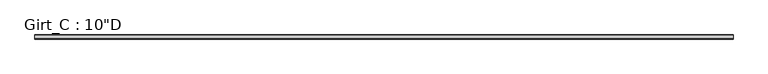
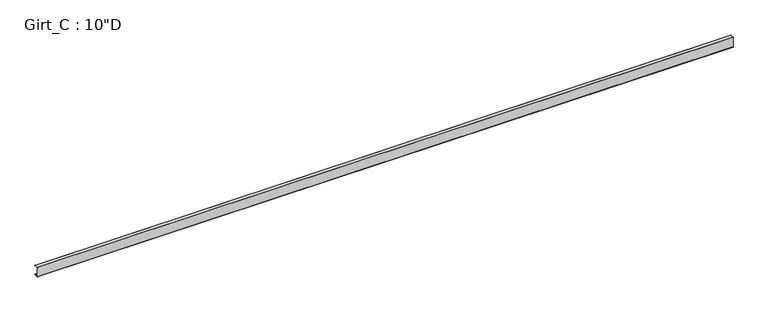
"""IFC4 building model written with IfcOpenShell, lengths in millimetres: beam geometry."""

import ifcopenshell
import ifcopenshell.guid

model = None  # the IFC model being written
_history = None  # IfcOwnerHistory: only IFC2X3 demands one
_inside = {}  # id of a spatial element -> (the spatial element, [elements in it])
_under = {}  # id of a project, library or spatial element -> (it, [spatial elements below it])
_declared = {}  # id of a project -> (the project, [libraries it declares])
_typed = {}  # id of a type object -> (the type object, [elements of that type])
_made_of = {}  # id of a material, layer set ... -> (it, [elements and type objects made of it])


def new_model(schema):
    """Start an empty IFC model of exactly this schema.

    Asked for "IFC4X3", IfcOpenShell would pick the latest addendum, in which some entities
    have other attributes; the version numbers below select the first issue.
    IFC2X3 requires an IfcOwnerHistory on every rooted entity: one is made here for all.
    """
    global model, _history
    if schema == "IFC4X3":
        model = ifcopenshell.file(schema_version=(4, 3, 0, 0))
    else:
        model = ifcopenshell.file(schema=schema)
    _inside.clear()
    _under.clear()
    _declared.clear()
    _typed.clear()
    _made_of.clear()
    _history = None
    if model.schema == "IFC2X3":
        org = make("IfcOrganization", Name="unknown")
        user = make(
            "IfcPersonAndOrganization",
            ThePerson=make("IfcPerson", FamilyName="unknown"),
            TheOrganization=org,
        )
        app = make(
            "IfcApplication",
            ApplicationDeveloper=org,
            Version="unknown",
            ApplicationFullName="unknown",
            ApplicationIdentifier="unknown",
        )
        _history = make(
            "IfcOwnerHistory",
            OwningUser=user,
            OwningApplication=app,
            ChangeAction="ADDED",
            CreationDate=0,
        )
    return model


def make(cls, **values):
    """One entity of the class cls with the attributes given. An attribute that is None is left unset."""
    return model.create_entity(
        cls, **{name: value for name, value in values.items() if value is not None}
    )


def rooted(cls, **values):
    """An entity with a GlobalId (a new one), such as an element, a storey or a relation."""
    return make(cls, GlobalId=ifcopenshell.guid.new(), OwnerHistory=_history, **values)


def si_unit(unit_type, name, prefix=None):
    """IfcSIUnit, for example si_unit("LENGTHUNIT", "METRE", prefix="MILLI")."""
    return make("IfcSIUnit", UnitType=unit_type, Prefix=prefix, Name=name)


def assignment(units):
    """IfcUnitAssignment: the units of a project."""
    return None if units is None else make("IfcUnitAssignment", Units=units)


def point(xyz):
    """IfcCartesianPoint."""
    return None if xyz is None else make("IfcCartesianPoint", Coordinates=xyz)


def direction(xyz):
    """IfcDirection."""
    return None if xyz is None else make("IfcDirection", DirectionRatios=xyz)


def frame(location, z_axis=None, x_axis=None):
    """IfcAxis2Placement3D, a coordinate frame: its origin and axes. An axis left out is left unset."""
    return make(
        "IfcAxis2Placement3D",
        Location=point(location),
        Axis=direction(z_axis),
        RefDirection=direction(x_axis),
    )


def frame_2d(location, x_axis=None):
    """IfcAxis2Placement2D, a coordinate frame in the plane: its origin and x axis."""
    return make(
        "IfcAxis2Placement2D", Location=point(location), RefDirection=direction(x_axis)
    )


def origin():
    """The frame at (0, 0, 0) with its axes left unset."""
    return frame((0.0, 0.0, 0.0))


def place(relative_to, where):
    """IfcLocalPlacement: puts the frame where relative to a parent placement (None: the world)."""
    return make(
        "IfcLocalPlacement", PlacementRelTo=relative_to, RelativePlacement=where
    )


def context(
    kind, dimensions, precision=None, world=None, true_north=None, identifier=None
):
    """IfcGeometricRepresentationContext, for example the 3D "Model" context."""
    return make(
        "IfcGeometricRepresentationContext",
        ContextIdentifier=identifier,
        ContextType=kind,
        CoordinateSpaceDimension=dimensions,
        Precision=precision,
        WorldCoordinateSystem=world,
        TrueNorth=true_north,
    )


def project(units=None, contexts=None):
    """IfcProject with its units and contexts."""
    return rooted(
        "IfcProject",
        Name="project",
        RepresentationContexts=contexts,
        UnitsInContext=assignment(units),
    )


def spatial(cls, under=None, at=None, **own):
    """A site, building, storey or space (cls), placed at a placement, below another one or the project."""
    s = rooted(cls, ObjectPlacement=at, **own)
    if under is not None:
        _under.setdefault(under.id(), (under, []))[1].append(s)
    return s


def polyline(points):
    """IfcPolyline through the points."""
    return make("IfcPolyline", Points=[point(p) for p in points])


def circle_curve(where, radius):
    """IfcCircle in the frame where."""
    return make("IfcCircle", Position=where, Radius=radius)


def trimmed(basis, trim1, trim2, sense, master):
    """IfcTrimmedCurve: the piece of a basis curve between two trims."""
    return make(
        "IfcTrimmedCurve",
        BasisCurve=basis,
        Trim1=trim1,
        Trim2=trim2,
        SenseAgreement=sense,
        MasterRepresentation=master,
    )


def segment(curve, same_sense, transition):
    """IfcCompositeCurveSegment."""
    return make(
        "IfcCompositeCurveSegment",
        Transition=transition,
        SameSense=same_sense,
        ParentCurve=curve,
    )


def composite_curve(segments, self_intersect=None):
    """IfcCompositeCurve: segments joined end to end."""
    return make("IfcCompositeCurve", Segments=segments, SelfIntersect=self_intersect)


def outline(outer, holes=None, kind="AREA"):
    """IfcArbitraryClosedProfileDef: a profile drawn as a closed curve; with holes, ...WithVoids."""
    if holes is None:
        return make("IfcArbitraryClosedProfileDef", ProfileType=kind, OuterCurve=outer)
    return make(
        "IfcArbitraryProfileDefWithVoids",
        ProfileType=kind,
        OuterCurve=outer,
        InnerCurves=holes,
    )


def extrude(swept, where, along, depth):
    """IfcExtrudedAreaSolid: the profile swept, set in the frame where, extruded along a direction by depth."""
    return make(
        "IfcExtrudedAreaSolid",
        SweptArea=swept,
        Position=where,
        ExtrudedDirection=direction(along),
        Depth=depth,
    )


def shape(context_of_items, identifier, shape_type, items):
    """IfcShapeRepresentation: the items that make up one representation, for example the "Body"."""
    return make(
        "IfcShapeRepresentation",
        ContextOfItems=context_of_items,
        RepresentationIdentifier=identifier,
        RepresentationType=shape_type,
        Items=items,
    )


def source(mapping_origin, context_of_items, identifier, shape_type, items):
    """IfcRepresentationMap: a shape defined once, which mapped items show again and again."""
    return make(
        "IfcRepresentationMap",
        MappingOrigin=mapping_origin,
        MappedRepresentation=shape(context_of_items, identifier, shape_type, items),
    )


def transform(
    local_origin,
    x_axis=None,
    y_axis=None,
    z_axis=None,
    scale=None,
    scale2=None,
    scale3=None,
    uniform=True,
):
    """IfcCartesianTransformationOperator3D, or its non-uniform kind. x_axis, y_axis, z_axis: its Axis1, 2, 3."""
    if uniform:
        return make(
            "IfcCartesianTransformationOperator3D",
            Axis1=direction(x_axis),
            Axis2=direction(y_axis),
            LocalOrigin=point(local_origin),
            Scale=scale,
            Axis3=direction(z_axis),
        )
    return make(
        "IfcCartesianTransformationOperator3DnonUniform",
        Axis1=direction(x_axis),
        Axis2=direction(y_axis),
        LocalOrigin=point(local_origin),
        Scale=scale,
        Axis3=direction(z_axis),
        Scale2=scale2,
        Scale3=scale3,
    )


def mapped(mapping_source, mapping_target):
    """IfcMappedItem: shows the shape of a source again, moved by a transform."""
    return make(
        "IfcMappedItem", MappingSource=mapping_source, MappingTarget=mapping_target
    )


def made_of(thing, what):
    """Note that an element or type object is made of a material, layer set ...; save() writes the relation."""
    if what is not None:
        _made_of.setdefault(what.id(), (what, []))[1].append(thing)
    return thing


def element(
    cls,
    number,
    at=None,
    inside=None,
    cuts=None,
    type_object=None,
    material=None,
    context=None,
    identifier="Body",
    shape_type=None,
    held_by="IfcProductDefinitionShape",
    body=None,
    shapes=None,
    **own,
):
    """One element of the class cls, such as IfcWall. Its Tag is "e" and its number.

    at: its placement. inside: the storey or other place that contains it. cuts: it is an
    opening in that element (IfcRelVoidsElement). A single representation is given by context,
    identifier, shape_type and body (its items); several are given by shapes. held_by: the class
    of the entity that holds the representations. save() writes the other relations.
    """
    e = rooted(cls, Tag="e%d" % number, ObjectPlacement=at, **own)
    if body is not None:
        shapes = [shape(context, identifier, shape_type, body)]
    if shapes is not None:
        e.Representation = make(held_by, Representations=shapes)
    if inside is not None:
        _inside.setdefault(inside.id(), (inside, []))[1].append(e)
    if cuts is not None:
        rooted(
            "IfcRelVoidsElement", RelatingBuildingElement=cuts, RelatedOpeningElement=e
        )
    if type_object is not None:
        _typed.setdefault(type_object.id(), (type_object, []))[1].append(e)
    return made_of(e, material)


def aggregate(whole, parts):
    """IfcRelAggregates: a whole, such as a stair, and the parts it consists of."""
    return rooted("IfcRelAggregates", RelatingObject=whole, RelatedObjects=parts)


def save(model, path):
    """Write the relations noted so far, then the file.

    IfcRelAggregates (storeys below a building ...), IfcRelContainedInSpatialStructure (elements
    in a storey), IfcRelDefinesByType, IfcRelAssociatesMaterial and IfcRelDeclares: one each for
    every whole, place, type object, material and project.
    """
    for whole, parts in _under.values():
        aggregate(whole, parts)
    for where, things in _inside.values():
        rooted(
            "IfcRelContainedInSpatialStructure",
            RelatedElements=things,
            RelatingStructure=where,
        )
    for kind, things in _typed.values():
        rooted("IfcRelDefinesByType", RelatedObjects=things, RelatingType=kind)
    for what, things in _made_of.values():
        rooted("IfcRelAssociatesMaterial", RelatedObjects=things, RelatingMaterial=what)
    for by, libraries in _declared.values():
        rooted("IfcRelDeclares", RelatingContext=by, RelatedDefinitions=libraries)
    model.write(path)


def beam_473ee45a(model_context):
    return source(origin(), model_context, "Body", "SweptSolid", [
        extrude(outline(composite_curve([segment(polyline([(87.5109375, 127.0), (99.7560415, 112.4068534), (97.6278742, 110.621109), (86.2154765, 124.221875), (3.3005807, 124.221875)]), True, "CONTINUOUS"), segment(trimmed(circle_curve(frame_2d((3.3741066, 122.2381931)), 1.9850441), [point((3.3005807, 124.221875))], [point((1.3890625, 122.2381931))], True, "CARTESIAN"), True, "CONTINUOUS"), segment(polyline([(1.3890625, 122.2381931), (1.3890625, -122.2389339)]), True, "CONTINUOUS"), segment(trimmed(circle_curve(frame_2d((3.3748024, -122.2389339)), 1.9857399), [point((1.3890625, -122.2389339))], [point((3.2694106, -124.221875))], True, "CARTESIAN"), True, "CONTINUOUS"), segment(polyline([(3.2694106, -124.221875), (86.2154765, -124.221875), (97.6510975, -110.5934327), (99.7792647, -112.379177), (87.5109375, -127.0), (3.3734375, -127.0)]), True, "CONTINUOUS"), segment(trimmed(circle_curve(frame_2d((3.3734375, -122.2375)), 4.7625), [point((3.3734375, -127.0))], [point((-1.3890625, -122.2375))], False, "CARTESIAN"), True, "CONTINUOUS"), segment(polyline([(-1.3890625, -122.2375), (-1.3890625, 122.2375)]), True, "CONTINUOUS"), segment(trimmed(circle_curve(frame_2d((3.3734375, 122.2375)), 4.7625), [point((-1.3890625, 122.2375))], [point((3.3734375, 127.0))], False, "CARTESIAN"), True, "CONTINUOUS"), segment(polyline([(3.3734375, 127.0), (87.5109375, 127.0)]), True, "CONTINUOUS")], self_intersect=False)), frame((-8465.6549, 0.0, 0.0), z_axis=(1.0, 0.0, 0.0), x_axis=(0.0, 1.0, 0.0)), (0.0, 0.0, 1.0), 16928.338),
    ])


if __name__ == "__main__":
    model = new_model("IFC4")
    model_context = context("Model", 3, world=origin())
    ifc_project = project(units=[si_unit("LENGTHUNIT", "METRE", prefix="MILLI")], contexts=[model_context])
    site = spatial("IfcSite", under=ifc_project)
    building = spatial("IfcBuilding", under=site)
    placement = place(None, origin())
    beam_shape = beam_473ee45a(model_context)
    element("IfcBeam", 1, ObjectType="Girt_C : 10\"D", at=placement, inside=building, context=model_context, shape_type="MappedRepresentation", body=[
        mapped(beam_shape, transform((0.0, 0.0, 0.0), x_axis=(1.0, 0.0, 0.0), y_axis=(0.0, 1.0, 0.0), z_axis=(0.0, 0.0, 1.0))),
    ])
    save(model, "model.ifc")

# Revit data of these elements
# Type "Girt_C : 10\"D"
#   half leg = 0' - 1 3/4"
#   Web_Thickness = 0' - 0 7/64"
#   Length [instance default] = 10' - 0"
#   Leg_1 = 0' - 3 1/2"
#   Height = 0' - 10"
#   Structural Material [instance default] = none
